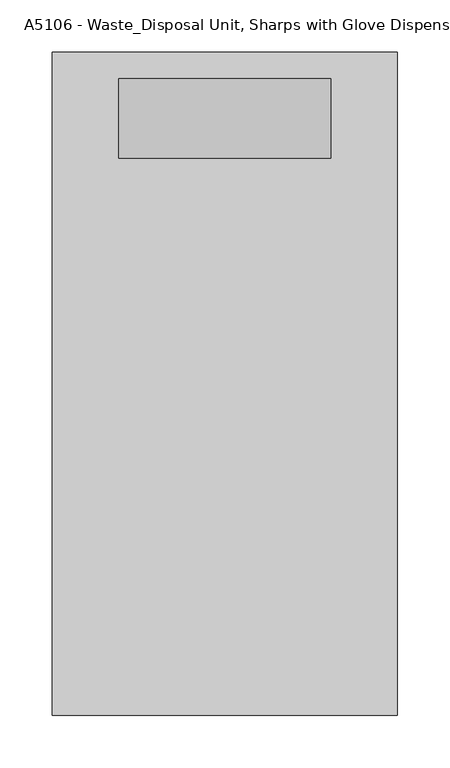
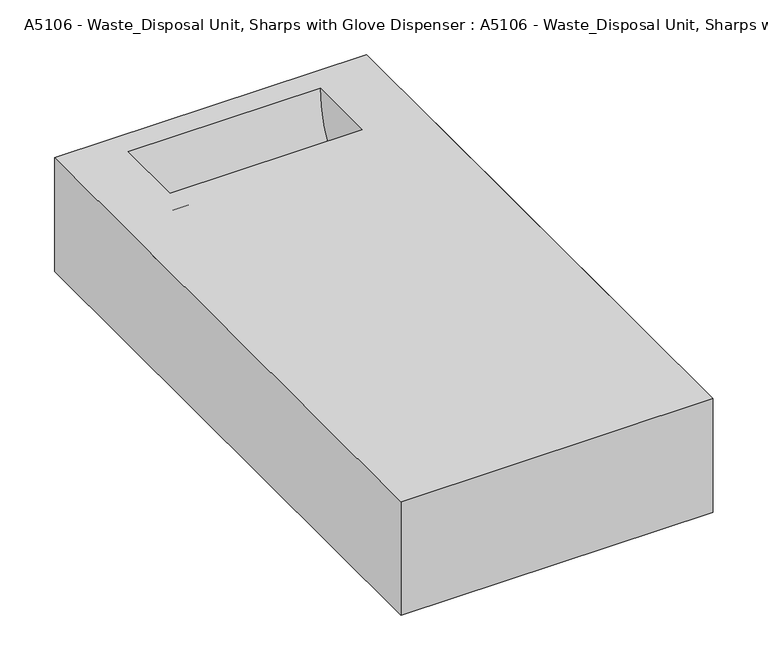
"""IFC4 building model written with IfcOpenShell, lengths in millimetres: proxy geometry, A5106 - Waste_Disposal Unit, Sharps with Glove Dispenser : A5106 - Waste_Disposal Unit, Sharps with Glove Dispenser."""

import ifcopenshell
import ifcopenshell.guid

model = None  # the IFC model being written
_history = None  # IfcOwnerHistory: only IFC2X3 demands one
_inside = {}  # id of a spatial element -> (the spatial element, [elements in it])
_under = {}  # id of a project, library or spatial element -> (it, [spatial elements below it])
_declared = {}  # id of a project -> (the project, [libraries it declares])
_typed = {}  # id of a type object -> (the type object, [elements of that type])
_made_of = {}  # id of a material, layer set ... -> (it, [elements and type objects made of it])


def new_model(schema):
    """Start an empty IFC model of exactly this schema.

    Asked for "IFC4X3", IfcOpenShell would pick the latest addendum, in which some entities
    have other attributes; the version numbers below select the first issue.
    IFC2X3 requires an IfcOwnerHistory on every rooted entity: one is made here for all.
    """
    global model, _history
    if schema == "IFC4X3":
        model = ifcopenshell.file(schema_version=(4, 3, 0, 0))
    else:
        model = ifcopenshell.file(schema=schema)
    _inside.clear()
    _under.clear()
    _declared.clear()
    _typed.clear()
    _made_of.clear()
    _history = None
    if model.schema == "IFC2X3":
        org = make("IfcOrganization", Name="unknown")
        user = make(
            "IfcPersonAndOrganization",
            ThePerson=make("IfcPerson", FamilyName="unknown"),
            TheOrganization=org,
        )
        app = make(
            "IfcApplication",
            ApplicationDeveloper=org,
            Version="unknown",
            ApplicationFullName="unknown",
            ApplicationIdentifier="unknown",
        )
        _history = make(
            "IfcOwnerHistory",
            OwningUser=user,
            OwningApplication=app,
            ChangeAction="ADDED",
            CreationDate=0,
        )
    return model


def make(cls, **values):
    """One entity of the class cls with the attributes given. An attribute that is None is left unset."""
    return model.create_entity(
        cls, **{name: value for name, value in values.items() if value is not None}
    )


def rooted(cls, **values):
    """An entity with a GlobalId (a new one), such as an element, a storey or a relation."""
    return make(cls, GlobalId=ifcopenshell.guid.new(), OwnerHistory=_history, **values)


def si_unit(unit_type, name, prefix=None):
    """IfcSIUnit, for example si_unit("LENGTHUNIT", "METRE", prefix="MILLI")."""
    return make("IfcSIUnit", UnitType=unit_type, Prefix=prefix, Name=name)


def assignment(units):
    """IfcUnitAssignment: the units of a project."""
    return None if units is None else make("IfcUnitAssignment", Units=units)


def point(xyz):
    """IfcCartesianPoint."""
    return None if xyz is None else make("IfcCartesianPoint", Coordinates=xyz)


def direction(xyz):
    """IfcDirection."""
    return None if xyz is None else make("IfcDirection", DirectionRatios=xyz)


def frame(location, z_axis=None, x_axis=None):
    """IfcAxis2Placement3D, a coordinate frame: its origin and axes. An axis left out is left unset."""
    return make(
        "IfcAxis2Placement3D",
        Location=point(location),
        Axis=direction(z_axis),
        RefDirection=direction(x_axis),
    )


def origin():
    """The frame at (0, 0, 0) with its axes left unset."""
    return frame((0.0, 0.0, 0.0))


def origin_with_axes():
    """The frame at (0, 0, 0) with the z axis (0, 0, 1) and the x axis (1, 0, 0) written out."""
    return frame((0.0, 0.0, 0.0), z_axis=(0.0, 0.0, 1.0), x_axis=(1.0, 0.0, 0.0))


def place(relative_to, where):
    """IfcLocalPlacement: puts the frame where relative to a parent placement (None: the world)."""
    return make(
        "IfcLocalPlacement", PlacementRelTo=relative_to, RelativePlacement=where
    )


def context(
    kind, dimensions, precision=None, world=None, true_north=None, identifier=None
):
    """IfcGeometricRepresentationContext, for example the 3D "Model" context."""
    return make(
        "IfcGeometricRepresentationContext",
        ContextIdentifier=identifier,
        ContextType=kind,
        CoordinateSpaceDimension=dimensions,
        Precision=precision,
        WorldCoordinateSystem=world,
        TrueNorth=true_north,
    )


def project(units=None, contexts=None):
    """IfcProject with its units and contexts."""
    return rooted(
        "IfcProject",
        Name="project",
        RepresentationContexts=contexts,
        UnitsInContext=assignment(units),
    )


def spatial(cls, under=None, at=None, **own):
    """A site, building, storey or space (cls), placed at a placement, below another one or the project."""
    s = rooted(cls, ObjectPlacement=at, **own)
    if under is not None:
        _under.setdefault(under.id(), (under, []))[1].append(s)
    return s


def polyline(points):
    """IfcPolyline through the points."""
    return make("IfcPolyline", Points=[point(p) for p in points])


def circle_curve(where, radius):
    """IfcCircle in the frame where."""
    return make("IfcCircle", Position=where, Radius=radius)


def outline(outer, holes=None, kind="AREA"):
    """IfcArbitraryClosedProfileDef: a profile drawn as a closed curve; with holes, ...WithVoids."""
    if holes is None:
        return make("IfcArbitraryClosedProfileDef", ProfileType=kind, OuterCurve=outer)
    return make(
        "IfcArbitraryProfileDefWithVoids",
        ProfileType=kind,
        OuterCurve=outer,
        InnerCurves=holes,
    )


def extrude(swept, where, along, depth):
    """IfcExtrudedAreaSolid: the profile swept, set in the frame where, extruded along a direction by depth."""
    return make(
        "IfcExtrudedAreaSolid",
        SweptArea=swept,
        Position=where,
        ExtrudedDirection=direction(along),
        Depth=depth,
    )


def shape(context_of_items, identifier, shape_type, items):
    """IfcShapeRepresentation: the items that make up one representation, for example the "Body"."""
    return make(
        "IfcShapeRepresentation",
        ContextOfItems=context_of_items,
        RepresentationIdentifier=identifier,
        RepresentationType=shape_type,
        Items=items,
    )


def source(mapping_origin, context_of_items, identifier, shape_type, items):
    """IfcRepresentationMap: a shape defined once, which mapped items show again and again."""
    return make(
        "IfcRepresentationMap",
        MappingOrigin=mapping_origin,
        MappedRepresentation=shape(context_of_items, identifier, shape_type, items),
    )


def transform(
    local_origin,
    x_axis=None,
    y_axis=None,
    z_axis=None,
    scale=None,
    scale2=None,
    scale3=None,
    uniform=True,
):
    """IfcCartesianTransformationOperator3D, or its non-uniform kind. x_axis, y_axis, z_axis: its Axis1, 2, 3."""
    if uniform:
        return make(
            "IfcCartesianTransformationOperator3D",
            Axis1=direction(x_axis),
            Axis2=direction(y_axis),
            LocalOrigin=point(local_origin),
            Scale=scale,
            Axis3=direction(z_axis),
        )
    return make(
        "IfcCartesianTransformationOperator3DnonUniform",
        Axis1=direction(x_axis),
        Axis2=direction(y_axis),
        LocalOrigin=point(local_origin),
        Scale=scale,
        Axis3=direction(z_axis),
        Scale2=scale2,
        Scale3=scale3,
    )


def mapped(mapping_source, mapping_target):
    """IfcMappedItem: shows the shape of a source again, moved by a transform."""
    return make(
        "IfcMappedItem", MappingSource=mapping_source, MappingTarget=mapping_target
    )


def made_of(thing, what):
    """Note that an element or type object is made of a material, layer set ...; save() writes the relation."""
    if what is not None:
        _made_of.setdefault(what.id(), (what, []))[1].append(thing)
    return thing


def element(
    cls,
    number,
    at=None,
    inside=None,
    cuts=None,
    type_object=None,
    material=None,
    context=None,
    identifier="Body",
    shape_type=None,
    held_by="IfcProductDefinitionShape",
    body=None,
    shapes=None,
    **own,
):
    """One element of the class cls, such as IfcWall. Its Tag is "e" and its number.

    at: its placement. inside: the storey or other place that contains it. cuts: it is an
    opening in that element (IfcRelVoidsElement). A single representation is given by context,
    identifier, shape_type and body (its items); several are given by shapes. held_by: the class
    of the entity that holds the representations. save() writes the other relations.
    """
    e = rooted(cls, Tag="e%d" % number, ObjectPlacement=at, **own)
    if body is not None:
        shapes = [shape(context, identifier, shape_type, body)]
    if shapes is not None:
        e.Representation = make(held_by, Representations=shapes)
    if inside is not None:
        _inside.setdefault(inside.id(), (inside, []))[1].append(e)
    if cuts is not None:
        rooted(
            "IfcRelVoidsElement", RelatingBuildingElement=cuts, RelatedOpeningElement=e
        )
    if type_object is not None:
        _typed.setdefault(type_object.id(), (type_object, []))[1].append(e)
    return made_of(e, material)


def aggregate(whole, parts):
    """IfcRelAggregates: a whole, such as a stair, and the parts it consists of."""
    return rooted("IfcRelAggregates", RelatingObject=whole, RelatedObjects=parts)


def save(model, path):
    """Write the relations noted so far, then the file.

    IfcRelAggregates (storeys below a building ...), IfcRelContainedInSpatialStructure (elements
    in a storey), IfcRelDefinesByType, IfcRelAssociatesMaterial and IfcRelDeclares: one each for
    every whole, place, type object, material and project.
    """
    for whole, parts in _under.values():
        aggregate(whole, parts)
    for where, things in _inside.values():
        rooted(
            "IfcRelContainedInSpatialStructure",
            RelatedElements=things,
            RelatingStructure=where,
        )
    for kind, things in _typed.values():
        rooted("IfcRelDefinesByType", RelatedObjects=things, RelatingType=kind)
    for what, things in _made_of.values():
        rooted("IfcRelAssociatesMaterial", RelatedObjects=things, RelatingMaterial=what)
    for by, libraries in _declared.values():
        rooted("IfcRelDeclares", RelatingContext=by, RelatedDefinitions=libraries)
    model.write(path)


def plane_surface(at):
    """IfcPlane: the flat surface through the origin of the frame at, square to its z axis."""
    return make("IfcPlane", Position=at)


def cylinder_surface(at, radius):
    """IfcCylindricalSurface: all points at the distance radius from the z axis of the frame at."""
    return make("IfcCylindricalSurface", Position=at, Radius=radius)


def revolved_surface(curve, axis_point, axis_direction):
    """IfcSurfaceOfRevolution: the curve turned about the line through axis_point along axis_direction."""
    return make(
        "IfcSurfaceOfRevolution",
        SweptCurve=make("IfcArbitraryOpenProfileDef", ProfileType="CURVE", Curve=curve),
        AxisPosition=make("IfcAxis1Placement", Location=point(axis_point), Axis=direction(axis_direction)),
    )


def advanced_brep(points, edges, surfaces, faces):
    """IfcAdvancedBrep: a solid bounded by faces that lie on surfaces and meet in shared edges.

    An edge is (start, end): straight between two places in points (the first is 0);
    or (start, end, curve); or (start, end, curve, False) where it runs against its curve.
    A face is (place in surfaces, loops), or (place, loops, False) where it looks against
    its surface's normal. A loop lists edges by number (the first is 1), with a minus sign
    where the edge is run from its end to its start. The first loop is the outer one.
    """
    corners = [point(p) for p in points]
    vertices = [make("IfcVertexPoint", VertexGeometry=c) for c in corners]
    made = []
    for start, end, *more in edges:
        made.append(
            make(
                "IfcEdgeCurve",
                EdgeStart=vertices[start],
                EdgeEnd=vertices[end],
                EdgeGeometry=more[0] if more else make("IfcPolyline", Points=[corners[start], corners[end]]),
                SameSense=more[1] if len(more) > 1 else True,
            )
        )
    hull = []
    for where, loops, *sense in faces:
        bounds = []
        for j, loop in enumerate(loops):
            ring = [make("IfcOrientedEdge", EdgeElement=made[abs(k) - 1], Orientation=k > 0) for k in loop]
            bounds.append(
                make(
                    "IfcFaceOuterBound" if j == 0 else "IfcFaceBound",
                    Bound=make("IfcEdgeLoop", EdgeList=ring),
                    Orientation=True,
                )
            )
        hull.append(make("IfcAdvancedFace", Bounds=bounds, FaceSurface=surfaces[where], SameSense=sense[0] if sense else True))
    return make("IfcAdvancedBrep", Outer=make("IfcClosedShell", CfsFaces=hull))


def a5106_waste_disposal_unit_sharps_with_glove_dispenser_a5106_6c6db77e(model_context):
    return source(origin(), model_context, "Body", "SolidModel", [
        advanced_brep(
        [(165.1, 558.8, 127.0), (-165.1, 558.8, 127.0), (-165.1, -76.2, 127.0), (165.1, -76.2, 127.0), (101.6, 533.4, 127.0), (101.6, 457.2, 127.0), (-101.6, 457.2, 127.0), (-101.6, 533.4, 127.0), (165.1, 558.8, 0.0), (165.1, -76.2, 0.0), (-165.1, -76.2, 0.0), (-165.1, 558.8, 0.0), (101.6, 457.2, 25.4), (-101.6, 457.2, 25.4)],
        [
            (0, 1),
            (1, 2),
            (2, 3),
            (3, 0),
            (4, 5),
            (5, 6),
            (6, 7),
            (7, 4),
            (8, 9),
            (9, 10),
            (10, 11),
            (11, 8),
            (0, 8),
            (11, 1),
            (10, 2),
            (9, 3),
            (4, 12, circle_curve(frame((101.6, 428.5291538, 126.2781346), z_axis=(-1.0, 0.0, 0.0), x_axis=(0.0, 1.0, 0.0)), 104.8733306)),
            (12, 5),
            (6, 13),
            (13, 7, circle_curve(frame((-101.6, 428.5291538, 126.2781346), z_axis=(1.0, 0.0, 0.0), x_axis=(0.0, 1.0, 0.0)), 104.8733306)),
            (12, 13),
        ],
        [
            plane_surface(frame((-165.1, 558.8, 127.0), z_axis=(0.0, 0.0, 1.0), x_axis=(-1.0, 0.0, 0.0))),
            plane_surface(frame((-165.1, 558.8, 0.0), z_axis=(0.0, 0.0, -1.0), x_axis=(1.0, 0.0, 0.0))),
            plane_surface(frame((165.1, 558.8, 127.0), z_axis=(0.0, 1.0, 0.0), x_axis=(0.0, 0.0, -1.0))),
            plane_surface(frame((-165.1, 558.8, 127.0), z_axis=(-1.0, 0.0, 0.0), x_axis=(0.0, 0.0, -1.0))),
            plane_surface(frame((-165.1, -76.2, 127.0), z_axis=(0.0, -1.0, 0.0), x_axis=(0.0, 0.0, -1.0))),
            plane_surface(frame((165.1, -76.2, 127.0), z_axis=(1.0, 0.0, 0.0), x_axis=(0.0, 0.0, -1.0))),
            plane_surface(frame((101.6, 457.2, 127.0), z_axis=(-1.0, 0.0, 0.0), x_axis=(0.0, 0.0, -1.0))),
            plane_surface(frame((-101.6, 457.2, 127.0), z_axis=(1.0, 0.0, 0.0), x_axis=(0.0, 0.0, 1.0))),
            plane_surface(frame((101.6, 457.2, 127.0), z_axis=(0.0, 1.0, 0.0), x_axis=(-1.0, 0.0, 0.0))),
            revolved_surface(polyline([(101.6, 533.4024844, 126.2781346), (-101.6, 533.4024844, 126.2781346)]), (-101.6, 428.5291538, 126.2781346), (1.0, 0.0, 0.0)),
        ],
        [
            (0, [[1, 2, 3, 4], [5, 6, 7, 8]]),
            (1, [[9, 10, 11, 12]]),
            (2, [[-1, 13, -12, 14]]),
            (3, [[-2, -14, -11, 15]]),
            (4, [[-3, -15, -10, 16]]),
            (5, [[-4, -16, -9, -13]]),
            (6, [[17, 18, -5]]),
            (7, [[19, 20, -7]]),
            (8, [[-18, 21, -19, -6]]),
            (9, [[-17, -8, -20, -21]]),
        ],
    ),
        advanced_brep(
        [(127.0, 431.8, 0.0), (127.0, 558.8, 127.0), (127.0, 431.8, 127.0), (-127.0, 431.8, 0.0), (-127.0, 431.8, 127.0), (-127.0, 558.8, 127.0), (101.6, 533.4, 127.0), (101.6, 457.2, 127.0), (-101.6, 457.2, 127.0), (-101.6, 533.4, 127.0), (101.6, 457.2, 25.4), (-101.6, 457.2, 25.4)],
        [
            (0, 1, circle_curve(frame((127.0, 431.8, 127.0), z_axis=(1.0, 0.0, 0.0), x_axis=(0.0, 0.0, -1.0)), 127.0)),
            (1, 2),
            (2, 0),
            (3, 4),
            (4, 5),
            (5, 3, circle_curve(frame((-127.0, 431.8, 127.0), z_axis=(-1.0, 0.0, 0.0), x_axis=(0.0, 0.0, -1.0)), 127.0)),
            (0, 3),
            (5, 1),
            (4, 2),
            (6, 7),
            (7, 8),
            (8, 9),
            (9, 6),
            (6, 10, circle_curve(frame((101.6, 428.5291538, 126.2781346), z_axis=(-1.0, 0.0, 0.0), x_axis=(0.0, 1.0, 0.0)), 104.8733306)),
            (10, 7),
            (8, 11),
            (11, 9, circle_curve(frame((-101.6, 428.5291538, 126.2781346), z_axis=(1.0, 0.0, 0.0), x_axis=(0.0, 1.0, 0.0)), 104.8733306)),
            (10, 11),
        ],
        [
            plane_surface(frame((127.0, 431.8, 0.0), z_axis=(1.0, 0.0, 0.0), x_axis=(0.0, 1.0, 0.0))),
            plane_surface(frame((-127.0, 431.8, 0.0), z_axis=(-1.0, 0.0, 0.0), x_axis=(0.0, -1.0, 0.0))),
            cylinder_surface(frame((-127.0, 431.8, 127.0), z_axis=(1.0, 0.0, 0.0), x_axis=(0.0, 0.0, -1.0)), 127.0),
            plane_surface(frame((127.0, 558.8, 127.0), z_axis=(0.0, 0.0, 1.0), x_axis=(-1.0, 0.0, 0.0))),
            plane_surface(frame((127.0, 431.8, 127.0), z_axis=(0.0, -1.0, 0.0), x_axis=(-1.0, 0.0, 0.0))),
            plane_surface(frame((101.6, 457.2, 127.0), z_axis=(-1.0, 0.0, 0.0), x_axis=(0.0, 0.0, -1.0))),
            plane_surface(frame((-101.6, 457.2, 127.0), z_axis=(1.0, 0.0, 0.0), x_axis=(0.0, 0.0, 1.0))),
            plane_surface(frame((101.6, 457.2, 127.0), z_axis=(0.0, 1.0, 0.0), x_axis=(-1.0, 0.0, 0.0))),
            revolved_surface(polyline([(101.6, 533.4024844, 126.2781346), (-101.6, 533.4024844, 126.2781346)]), (-101.6, 428.5291538, 126.2781346), (1.0, 0.0, 0.0)),
        ],
        [
            (0, [[1, 2, 3]]),
            (1, [[4, 5, 6]]),
            (2, [[-1, 7, -6, 8]]),
            (3, [[-2, -8, -5, 9], [10, 11, 12, 13]]),
            (4, [[-3, -9, -4, -7]]),
            (5, [[14, 15, -10]]),
            (6, [[16, 17, -12]]),
            (7, [[-15, 18, -16, -11]]),
            (8, [[-14, -13, -17, -18]]),
        ],
    ),
        extrude(outline(polyline([(127.0, 76.2), (127.0, -76.2), (-127.0, -76.2), (-127.0, 76.2), (127.0, 76.2)])), origin_with_axes(), (0.0, 0.0, 1.0), 101.6),
        extrude(outline(polyline([(165.1, 431.8), (165.1, 76.2), (-165.1, 76.2), (-165.1, 431.8), (165.1, 431.8)])), origin_with_axes(), (0.0, 0.0, 1.0), 127.0),
    ])


if __name__ == "__main__":
    model = new_model("IFC4")
    model_context = context("Model", 3, world=origin())
    ifc_project = project(units=[si_unit("LENGTHUNIT", "METRE", prefix="MILLI")], contexts=[model_context])
    site = spatial("IfcSite", under=ifc_project)
    building = spatial("IfcBuilding", under=site)
    placement = place(None, origin())
    a5106_waste_disposal_unit_sharps_with_glove_dispenser_a5106_shape = a5106_waste_disposal_unit_sharps_with_glove_dispenser_a5106_6c6db77e(model_context)
    element("IfcBuildingElementProxy", 1, Name="A5106 - Waste_Disposal Unit, Sharps with Glove Dispenser : A5106 - Waste_Disposal Unit, Sharps with Glove Dispenser", ObjectType="A5106 - Waste_Disposal Unit, Sharps with Glove Dispenser : A5106 - Waste_Disposal Unit, Sharps with Glove Dispenser", at=placement, inside=building, context=model_context, shape_type="MappedRepresentation", body=[
        mapped(a5106_waste_disposal_unit_sharps_with_glove_dispenser_a5106_shape, transform((0.0, 0.0, 0.0), x_axis=(1.0, 0.0, 0.0), y_axis=(0.0, 1.0, 0.0), z_axis=(0.0, 0.0, 1.0))),
    ])
    save(model, "model.ifc")

# Revit data of these elements
# Type "A5106 - Waste_Disposal Unit, Sharps with Glove Dispenser : A5106 - Waste_Disposal Unit, Sharps with Glove Dispenser"
#   Watts2 = "0"
#   Watts1 = "0"
#   Unit_Issue = "EA"
#   UTIL_6_Misc = "-"
#   UTIL_5_NonMedGas = "-"
#   UTIL_4_MiscGas = "-"
#   UTIL_3_MedGas = "-"
#   UTIL_2_Elec = "-"
#   UTIL_1_WaterDrain = "-"
#   Nomenclature = "Waste Disposal Unit, Sharps w/Glove Dispenser"
#   NSN = "6530"
#   Location [instance default] = ""
#   JSN = "A5106"
#   Fund_Source_VA = "-"
#   Fund_Source_Navy = "-"
#   Fund_Source_Army = "-"
#   Fund_Source_AF = "-"
#   ELEC_Volts2 = "0"
#   ELEC_Volts1 = "0"
#   ELEC_Phase2 = "0"
#   ELEC_Phase1 = "0"
#   ELEC_HertzSwitch = "0"
#   ELEC_HertzDependent = "0"
#   ELEC_Hertz = "0"
#   ELEC_Amps2 = "0"
#   ELEC_Amps1 = "0"
#   DetailDescription = "The unit is designed for the disposal of sharps and complies with OSHA guidelines for the handling of sharps. It shall house a 5 quart container and be capable of being mounted on a wall. It shall have a glove dispenser attached. The unit shall be secured by a locked enclosure."
#   CAT_VA = "C"
#   CAT_Navy = "A"
#   CAT_IHS = "-"
#   CAT_Army = "C"
#   CAT_AF = "C"
#   BTUperhour = "0"
#   Weight_IP = 5
#   Default Elevation = 4' - 0"
#   DIM_Width_IP = 1' - 1"
#   DIM_Height_IP = 2' - 1"
#   DIM_Depth_IP = 0' - 5"
#   finish [instance default] = none
#   Assembly Code = ""
# Element 1 (IfcBuildingElementProxy, "A5106 - Waste_Disposal Unit, Sharps with Glove Dispenser : A5106 - Waste_Disposal Unit, Sharps with Glove Dispenser")
#   Materials on its faces: "EquipSpace"
# Materials
#   "EquipSpace": class "Unassigned", colour RGB 221 217 195, transparency 0.5
